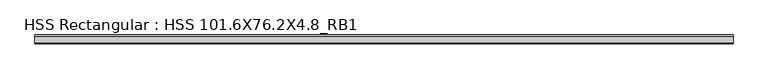
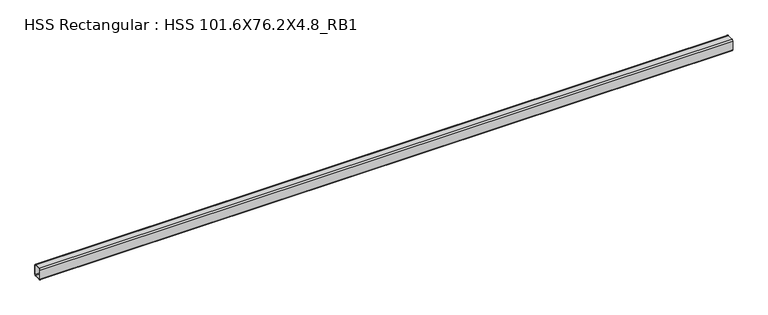
"""IFC4 building model written with IfcOpenShell, lengths in millimetres: beam geometry, HSS Rectangular : HSS 101.6X76.2X4.8_RB1."""

from ifc_helpers import new_model, si_unit, point, frame, frame_2d, origin, place, context, project, spatial, polyline, circle_curve, trimmed, segment, composite_curve, outline, extrude, source, transform, mapped, element, save


def hss_rectangular_hss_101_6x76_2x4_8_rb1_bebc4ede(model_context):
    return source(origin(), model_context, "Body", "SweptSolid", [
        extrude(outline(composite_curve([segment(polyline([(38.1, 41.275), (38.1, -41.275)]), True, "CONTINUOUS"), segment(trimmed(circle_curve(frame_2d((28.575, -41.275)), 9.525), [point((38.1, -41.275))], [point((28.575, -50.8))], False, "CARTESIAN"), True, "CONTINUOUS"), segment(polyline([(28.575, -50.8), (-28.575, -50.8)]), True, "CONTINUOUS"), segment(trimmed(circle_curve(frame_2d((-28.575, -41.275)), 9.525), [point((-28.575, -50.8))], [point((-38.1, -41.275))], False, "CARTESIAN"), True, "CONTINUOUS"), segment(polyline([(-38.1, -41.275), (-38.1, 41.275)]), True, "CONTINUOUS"), segment(trimmed(circle_curve(frame_2d((-28.575, 41.275)), 9.525), [point((-38.1, 41.275))], [point((-28.575, 50.8))], False, "CARTESIAN"), True, "CONTINUOUS"), segment(polyline([(-28.575, 50.8), (28.575, 50.8)]), True, "CONTINUOUS"), segment(trimmed(circle_curve(frame_2d((28.575, 41.275)), 9.525), [point((28.575, 50.8))], [point((38.1, 41.275))], False, "CARTESIAN"), True, "CONTINUOUS")], self_intersect=False), holes=[composite_curve([segment(trimmed(circle_curve(frame_2d((-28.575, 41.275)), 4.7625), [point((-28.575, 46.0375))], [point((-33.3375, 41.275))], True, "CARTESIAN"), True, "CONTINUOUS"), segment(polyline([(-33.3375, 41.275), (-33.3375, -41.275)]), True, "CONTINUOUS"), segment(trimmed(circle_curve(frame_2d((-28.575, -41.275)), 4.7625), [point((-33.3375, -41.275))], [point((-28.575, -46.0375))], True, "CARTESIAN"), True, "CONTINUOUS"), segment(polyline([(-28.575, -46.0375), (28.575, -46.0375)]), True, "CONTINUOUS"), segment(trimmed(circle_curve(frame_2d((28.575, -41.275)), 4.7625), [point((28.575, -46.0375))], [point((33.3375, -41.275))], True, "CARTESIAN"), True, "CONTINUOUS"), segment(polyline([(33.3375, -41.275), (33.3375, 41.275)]), True, "CONTINUOUS"), segment(trimmed(circle_curve(frame_2d((28.575, 41.275)), 4.7625), [point((33.3375, 41.275))], [point((28.575, 46.0375))], True, "CARTESIAN"), True, "CONTINUOUS"), segment(polyline([(28.575, 46.0375), (-28.575, 46.0375)]), True, "CONTINUOUS")], self_intersect=False)]), frame((-7525.9966117, 0.0, 0.0), z_axis=(1.0, 0.0, 0.0), x_axis=(0.0, 1.0, 0.0)), (0.0, 0.0, 1.0), 5998.008198),
    ])


if __name__ == "__main__":
    model = new_model("IFC4")
    model_context = context("Model", 3, world=origin())
    ifc_project = project(units=[si_unit("LENGTHUNIT", "METRE", prefix="MILLI")], contexts=[model_context])
    site = spatial("IfcSite", under=ifc_project)
    building = spatial("IfcBuilding", under=site)
    placement = place(None, origin())
    hss_rectangular_hss_101_6x76_2x4_8_rb1_shape = hss_rectangular_hss_101_6x76_2x4_8_rb1_bebc4ede(model_context)
    element("IfcBeam", 1, ObjectType="HSS Rectangular : HSS 101.6X76.2X4.8_RB1", at=placement, inside=building, context=model_context, shape_type="MappedRepresentation", body=[
        mapped(hss_rectangular_hss_101_6x76_2x4_8_rb1_shape, transform((0.0, 0.0, 0.0), x_axis=(1.0, 0.0, 0.0), y_axis=(0.0, 1.0, 0.0), z_axis=(0.0, 0.0, 1.0))),
    ])
    save(model, "model.ifc")

# Revit data of these elements
# Type "HSS Rectangular : HSS 101.6X76.2X4.8_RB1"
#   Section Name Key = "HSS 4X3X3/16"
#   Assembly Code = "B10"
#   Width = 7.62 cm
#   Wall Nominal Thickness = 0.4763 cm
#   Wall Design Thickness = 0.442 cm
#   Torsional Moment of Inertia = 260.561 cm⁴
#   Torsional Modulus = 61.2876 cm³
#   Section Area = 14.4516 cm²
#   Plastic Modulus weak axis = 40.3122 cm³
#   Plastic Modulus strong axis = 49.1612 cm³
#   Perimeter = 0.881482 m²/m
#   Outer Fillet = 0.9525 cm
#   Nominal Weight = 12.1285 kgf/m
#   Moment of Inertia weak axis = 131.529 cm⁴
#   Moment of Inertia strong axis = 205.202 cm⁴
#   Inner Fillet = 0.4763 cm
#   Height = 10.16 cm
#   Elastic Modulus weak axis = 34.4128 cm³
#   Elastic Modulus strong axis = 40.476 cm³
#   Centroid Vertical = 5.08 cm
#   Centroid Horizontal = 3.81 cm
#   Length [instance default] = 1524 mm
#   Structural Material [instance default] = Steel ASTM A500, Grade B, Rectangular and Square
#   Principal Axes Angle = 0
# Element 1 (IfcBeam, "HSS Rectangular : HSS 101.6X76.2X4.8_RB1")
#   Structural Material = Steel ASTM A992
#   Materials on its faces: "Steel ASTM A992"
# Materials
#   "Steel ASTM A500, Grade B, Rectangular and Square": class "Metal", colour RGB 199 199 199, transparency 0, Description = "Carbon steel", Cost = 0
#   "Steel ASTM A992": class "Metal", colour RGB 199 199 199, transparency 0, Description = "Structural steel 50ksi", Cost = 0
